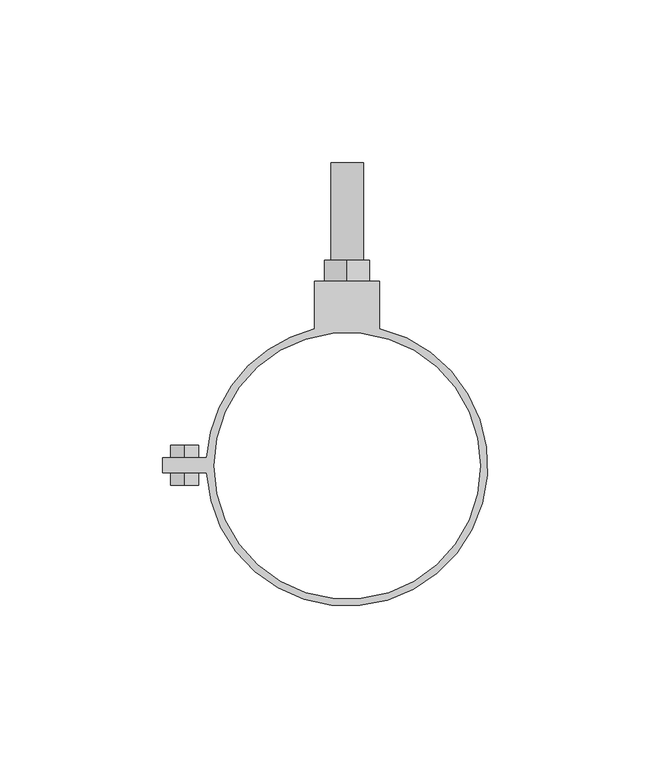
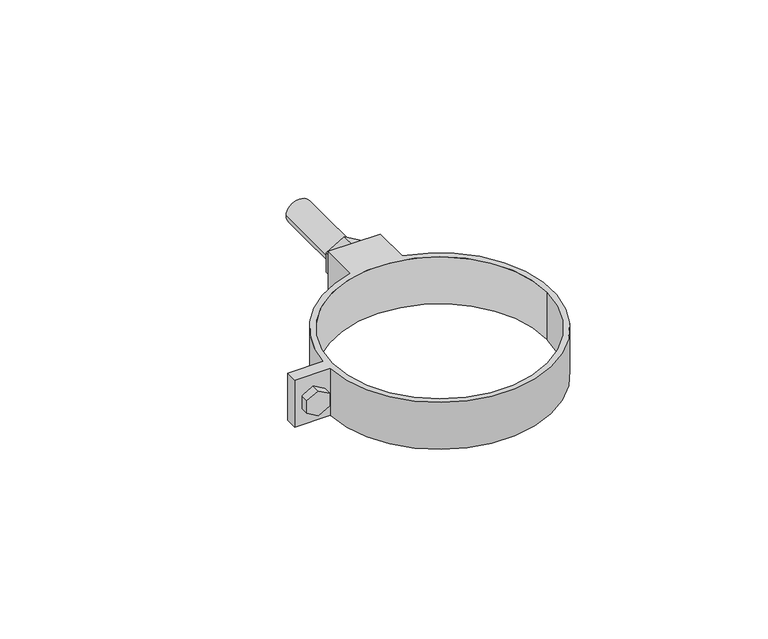
"""IFC4 building model written with IfcOpenShell, lengths in millimetres: proxy geometry, TN_ПВС 125-82_Хомут универсальный : TN_ПВС 125-82_Хомут универсальный."""

from ifc_helpers import new_model, si_unit, point, frame, frame_2d, origin, origin_2d, place, context, project, spatial, polyline, circle_curve, trimmed, segment, composite_curve, outline, extrude, source, transform, mapped, element, save


def generic_models_1d4bbf5b(model_context):
    return source(origin(), model_context, "Body", "SweptSolid", [
        extrude(outline(composite_curve([segment(trimmed(circle_curve(origin_2d(), 5.0), [point((0.0, -5.0))], [point((0.0, 5.0))], False, "CARTESIAN"), True, "CONTINUOUS"), segment(trimmed(circle_curve(origin_2d(), 5.0), [point((0.0, 5.0))], [point((0.0, -5.0))], False, "CARTESIAN"), True, "CONTINUOUS")], self_intersect=False)), frame((0.0, 56.8, 0.0), z_axis=(0.0, 1.0, 0.0), x_axis=(0.0, 0.0, 1.0)), (0.0, 0.0, 1.0), 36.5),
        extrude(outline(composite_curve([segment(trimmed(circle_curve(frame_2d((0.0024173, -0.0004914)), 43.3003134), [point((-43.2256543, 2.4997019))], [point((-9.9935423, 42.1302329))], False, "CARTESIAN"), True, "CONTINUOUS"), segment(polyline([(-9.9935423, 42.1302329), (-9.9935423, 56.8), (9.9935423, 56.8), (9.9935423, 42.2254395)]), True, "CONTINUOUS"), segment(trimmed(circle_curve(frame_2d((-0.0424661, 0.1408408)), 43.2647075), [point((9.9935423, 42.2254395))], [point((-43.2481974, -2.1174098))], False, "CARTESIAN"), True, "CONTINUOUS"), segment(polyline([(-43.2481974, -2.1174098), (-56.859662, -2.1174098), (-56.859662, 2.4997019), (-43.2256543, 2.4997019)]), True, "CONTINUOUS")], self_intersect=False), holes=[composite_curve([segment(trimmed(circle_curve(origin_2d(), 41.0), [point((-41.0, 0.0))], [point((41.0, 0.0))], True, "CARTESIAN"), True, "CONTINUOUS"), segment(trimmed(circle_curve(origin_2d(), 41.0), [point((41.0, 0.0))], [point((-41.0, 0.0))], True, "CARTESIAN"), True, "CONTINUOUS")], self_intersect=False)]), frame((0.0, 0.0, -9.5), z_axis=(0.0, 0.0, 1.0), x_axis=(1.0, 0.0, 0.0)), (0.0, 0.0, 1.0), 19.0),
        extrude(outline(polyline([(-4.006052, 6.9386855), (4.006052, 6.9386855), (8.0121039, 0.0), (4.006052, -6.9386855), (-4.006052, -6.9386855), (-8.0121039, 0.0), (-4.006052, 6.9386855)])), frame((0.0, 56.8, 0.0), z_axis=(0.0, 1.0, 0.0), x_axis=(0.0, 0.0, 1.0)), (0.0, 0.0, 1.0), 6.5),
        extrude(outline(polyline([(-2.5, -45.669873), (2.5, -45.669873), (5.0, -50.0), (2.5, -54.330127), (-2.5, -54.330127), (-5.0, -50.0), (-2.5, -45.669873)])), frame((0.0, -5.9452765, 0.0), z_axis=(0.0, 1.0, 0.0), x_axis=(0.0, 0.0, 1.0)), (0.0, 0.0, 1.0), 12.2367894),
    ])


if __name__ == "__main__":
    model = new_model("IFC4")
    model_context = context("Model", 3, world=origin())
    ifc_project = project(units=[si_unit("LENGTHUNIT", "METRE", prefix="MILLI")], contexts=[model_context])
    site = spatial("IfcSite", under=ifc_project)
    building = spatial("IfcBuilding", under=site)
    placement = place(None, origin())
    generic_models_shape = generic_models_1d4bbf5b(model_context)
    element("IfcBuildingElementProxy", 1, Name="TN_ПВС 125-82_Хомут универсальный : TN_ПВС 125-82_Хомут универсальный", ObjectType="TN_ПВС 125-82_Хомут универсальный : TN_ПВС 125-82_Хомут универсальный", at=placement, inside=building, context=model_context, shape_type="MappedRepresentation", body=[
        mapped(generic_models_shape, transform((0.0, 0.0, 0.0), x_axis=(1.0, 0.0, 0.0), y_axis=(0.0, 1.0, 0.0), z_axis=(0.0, 0.0, 1.0))),
    ])
    save(model, "model.ifc")

# Revit data of these elements
# Type "TN_ПВС 125-82_Хомут универсальный : TN_ПВС 125-82_Хомут универсальный"
#   Description = "Предназначен для крепления водосточной трубы на необходимом от фасада\r\nрасстоянии"
#   Manufacturer = "ТехноНИКОЛЬ"
#   Model = "Комплектующие к водосточным системам"
#   URL = "https://tn-vodostok.ru/catalog/pvh/"
#   ADSK_Обозначение = "ТехноНИКОЛЬ"
#   ADSK_Наименование краткое = "Хомут"
#   ADSK_Наименование = "Хомут универсальный"
#   ADSK_Масса_Текст = ""
#   ADSK_Марка = ""
#   ADSK_Код изделия = ""
#   ADSK_Завод-изготовитель = "ТехноНИКОЛЬ"
#   ADSK_Единица измерения = "шт."
#   ADSK_Группирование = "Комплектующие к водосточным системам"
#   ADSK_URL страницы изделия = "https://tn-vodostok.ru/catalog/pvh/"
#   ADSK_URL документации изделия = "https://tn-vodostok.ru/upload/iblock/c42/c427963cb77eb5c3c51f0cfb870e9e52.pdf"
#   ADSK_Размер_Диаметр = 82 mm
#   ADSK_Размер_Высота = 19 mm
#   ADSK_Количество = 1
#   ADSK_Материал [instance default] = TN_Пластик_Коричневый_RAL8019
#   Default Elevation = 0
# Element 1 (IfcBuildingElementProxy, "TN_ПВС 125-82_Хомут универсальный : TN_ПВС 125-82_Хомут универсальный")
#   Materials on its faces: "TN_Пластик_Коричневый_RAL8019", "TN_СтальГальванизированная_Серый"
# Materials
#   "TN_Пластик_Коричневый_RAL8019": class "Типовые", colour RGB 61 54 53, transparency 0, Cost = 0
#   "TN_СтальГальванизированная_Серый": class "Типовые", colour RGB 206 210 213, transparency 0, Cost = 0
